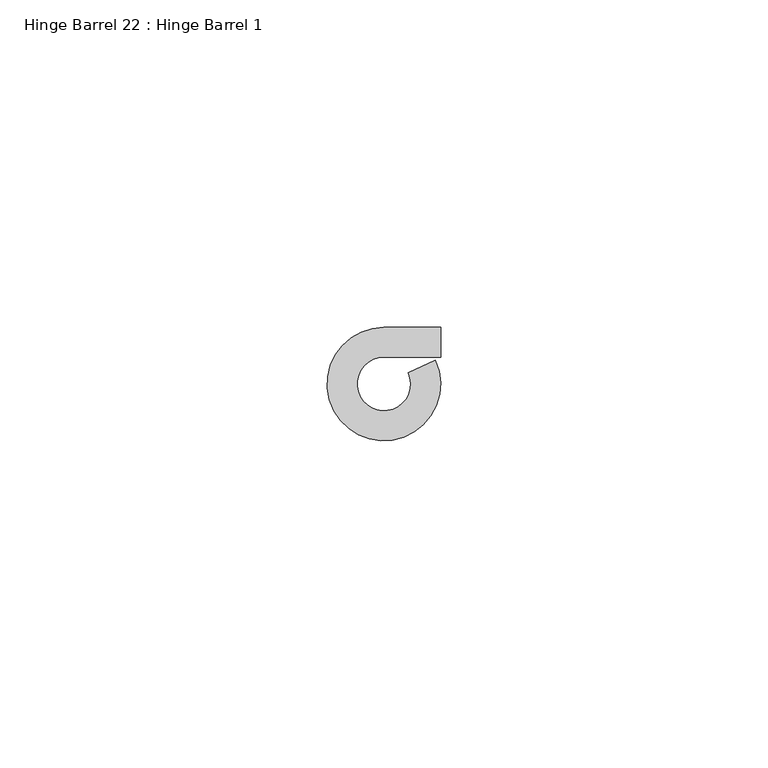
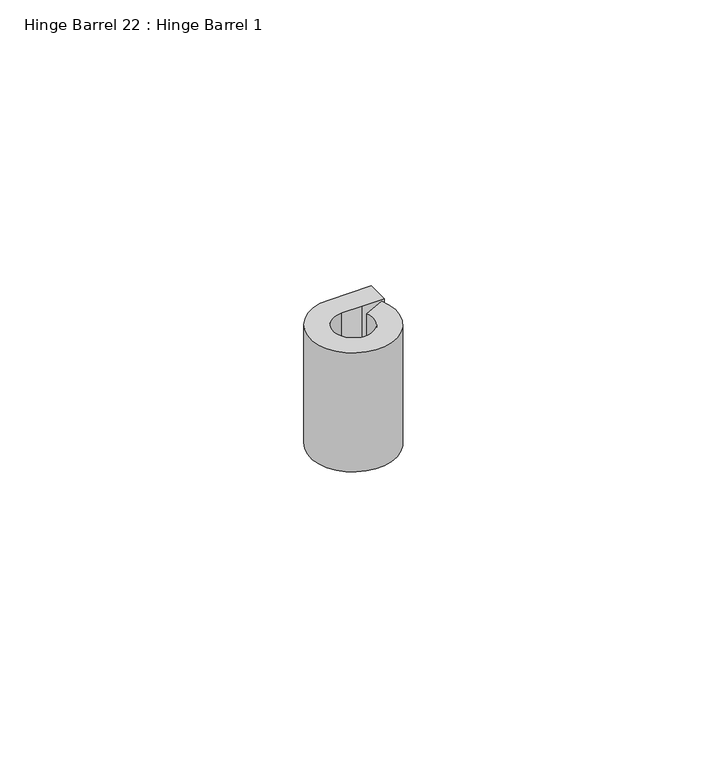
"""IFC4 building model written with IfcOpenShell, lengths in millimetres: proxy geometry, Hinge Barrel 22 : Hinge Barrel 1."""

from ifc_helpers import new_model, si_unit, point, frame, frame_2d, origin, place, context, project, spatial, polyline, circle_curve, trimmed, segment, composite_curve, outline, extrude, source, transform, mapped, element, save


def hinge_barrel_22_hinge_barrel_1_43aeb578(model_context):
    return source(origin(), model_context, "Body", "SweptSolid", [
        extrude(outline(composite_curve([segment(polyline([(587323.2214739, -533980.5883841), (587319.1320739, -533980.5883841)]), True, "CONTINUOUS"), segment(trimmed(circle_curve(frame_2d((587319.1320739, -533984.6777841)), 4.0894), [point((587319.1320739, -533980.5883841))], [point((587322.8436736, -533982.9610371))], True, "CARTESIAN"), True, "CONTINUOUS"), segment(polyline([(587322.8436736, -533982.9610371), (587326.986084, -533981.0450249)]), True, "CONTINUOUS"), segment(trimmed(circle_curve(frame_2d((587319.1320739, -533984.6777841)), 8.6534625), [point((587326.986084, -533981.0450249))], [point((587319.1320739, -533976.0243216))], False, "CARTESIAN"), True, "CONTINUOUS"), segment(polyline([(587319.1320739, -533976.0243216), (587327.7934739, -533976.0243216), (587327.7934739, -533980.5883841), (587323.2214739, -533980.5883841)]), True, "CONTINUOUS")], self_intersect=False)), frame((0.0, 0.0, 2038.35), z_axis=(0.0, 0.0, 1.0), x_axis=(1.0, 0.0, 0.0)), (0.0, 0.0, 1.0), 25.4),
    ])


if __name__ == "__main__":
    model = new_model("IFC4")
    model_context = context("Model", 3, world=origin())
    ifc_project = project(units=[si_unit("LENGTHUNIT", "METRE", prefix="MILLI")], contexts=[model_context])
    site = spatial("IfcSite", under=ifc_project)
    building = spatial("IfcBuilding", under=site)
    placement = place(None, origin())
    hinge_barrel_22_hinge_barrel_1_shape = hinge_barrel_22_hinge_barrel_1_43aeb578(model_context)
    element("IfcBuildingElementProxy", 1, Name="Hinge Barrel 22 : Hinge Barrel 1", ObjectType="Hinge Barrel 22 : Hinge Barrel 1", at=placement, inside=building, context=model_context, shape_type="MappedRepresentation", body=[
        mapped(hinge_barrel_22_hinge_barrel_1_shape, transform((0.0, 0.0, 0.0), x_axis=(1.0, 0.0, 0.0), y_axis=(0.0, 1.0, 0.0), z_axis=(0.0, 0.0, 1.0))),
    ])
    save(model, "model.ifc")

# Revit data of these elements
# Element 1 (IfcBuildingElementProxy, "Hinge Barrel 22 : Hinge Barrel 1")
#   Materials on its faces: "6\"X6\" WELD-ON STL BUTT HINGE"
# Materials
#   "6\"X6\" WELD-ON STL BUTT HINGE": class "Metal", colour RGB 189 187 185, transparency 0, Description = "Carbon steel", Cost = 0
